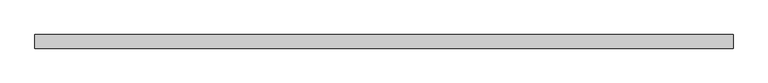
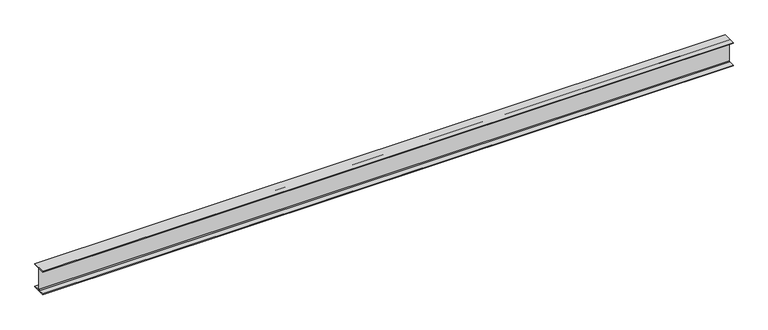
"""IFC4 building model written with IfcOpenShell, lengths in millimetres: beam geometry, Old_Steel Beam_H-KSD3502 : H_SB_ASB_H-390×300x10x16."""

from ifc_helpers import new_model, si_unit, point, frame, frame_2d, origin, place, context, project, spatial, polyline, circle_curve, trimmed, segment, composite_curve, outline, extrude, source, transform, mapped, element, save


def beam_f1becc55(model_context):
    return source(origin(), model_context, "Body", "SweptSolid", [
        extrude(outline(composite_curve([segment(polyline([(82.5, -141.5), (82.5, -151.7), (-82.5, -151.7), (-82.5, -141.5), (-11.9, -141.5)]), True, "CONTINUOUS"), segment(trimmed(circle_curve(frame_2d((-11.9, -132.6)), 8.9), [point((-11.9, -141.5))], [point((-3.0, -132.6))], True, "CARTESIAN"), True, "CONTINUOUS"), segment(polyline([(-3.0, -132.6), (-3.0, 132.6)]), True, "CONTINUOUS"), segment(trimmed(circle_curve(frame_2d((-11.9, 132.6)), 8.9), [point((-3.0, 132.6))], [point((-11.9, 141.5))], True, "CARTESIAN"), True, "CONTINUOUS"), segment(polyline([(-11.9, 141.5), (-82.5, 141.5), (-82.5, 151.7), (82.5, 151.7), (82.5, 141.5), (11.9, 141.5)]), True, "CONTINUOUS"), segment(trimmed(circle_curve(frame_2d((11.9, 132.6)), 8.9), [point((11.9, 141.5))], [point((3.0, 132.6))], True, "CARTESIAN"), True, "CONTINUOUS"), segment(polyline([(3.0, 132.6), (3.0, -132.6)]), True, "CONTINUOUS"), segment(trimmed(circle_curve(frame_2d((11.9, -132.6)), 8.9), [point((3.0, -132.6))], [point((11.9, -141.5))], True, "CARTESIAN"), True, "CONTINUOUS"), segment(polyline([(11.9, -141.5), (82.5, -141.5)]), True, "CONTINUOUS")], self_intersect=False)), frame((-4237.2999994, 0.0, 0.0), z_axis=(1.0, 0.0, 0.0), x_axis=(0.0, 1.0, 0.0)), (0.0, 0.0, 1.0), 8474.5999988),
    ])


if __name__ == "__main__":
    model = new_model("IFC4")
    model_context = context("Model", 3, world=origin())
    ifc_project = project(units=[si_unit("LENGTHUNIT", "METRE", prefix="MILLI")], contexts=[model_context])
    site = spatial("IfcSite", under=ifc_project)
    building = spatial("IfcBuilding", under=site)
    placement = place(None, origin())
    beam_shape = beam_f1becc55(model_context)
    element("IfcBeam", 1, ObjectType="Old_Steel Beam_H-KSD3502 : H_SB_ASB_H-390×300x10x16", at=placement, inside=building, context=model_context, shape_type="MappedRepresentation", body=[
        mapped(beam_shape, transform((0.0, 0.0, 0.0), x_axis=(1.0, 0.0, 0.0), y_axis=(0.0, 1.0, 0.0), z_axis=(0.0, 0.0, 1.0))),
    ])
    save(model, "model.ifc")

# Revit data of these elements
# Type "Old_Steel Beam_H-KSD3502 : H_SB_ASB_H-390×300x10x16"
#   Width = 30.0 cm
#   Web Thickness = 1.0 cm
#   Web Fillet = 2.2 cm
#   Warping Constant = 2517770.0 cm⁶
#   Torsional Moment of Inertia = 94.3867 cm⁴
#   Torsional Modulus = 1.0 cm³
#   Section Area = 136.0 cm²
#   Plastic Modulus weak axis = 733.0 cm³
#   Plastic Modulus strong axis = 2190.0 cm³
#   Perimeter = 1.92 m²/m
#   Nominal Weight = 107.00 kgf/m
#   Moment of Inertia weak axis = 7210.00 cm⁴
#   Moment of Inertia strong axis = 38700.00 cm⁴
#   Height = 39.0 cm
#   Flange Thickness = 1.6 cm
#   Elastic Modulus weak axis = 481.0 cm³
#   Elastic Modulus strong axis = 1980.0 cm³
#   Centroid Vertical = 19.5 cm
#   Centroid Horizontal = 15.0 cm
#   Length [instance default] = 1.5240 m
#   Structural Material [instance default] = Steel, 45-345
#   Assembly Code = ""
# Element 1 (IfcBeam, "Old_Steel Beam_H-KSD3502 : H_SB_ASB_H-390×300x10x16")
#   Structural Material = none
# Materials
#   "Steel, 45-345": class "Metal", colour RGB 189 187 185, transparency 0, Description = "Steel 345 MPa", Cost = 0
